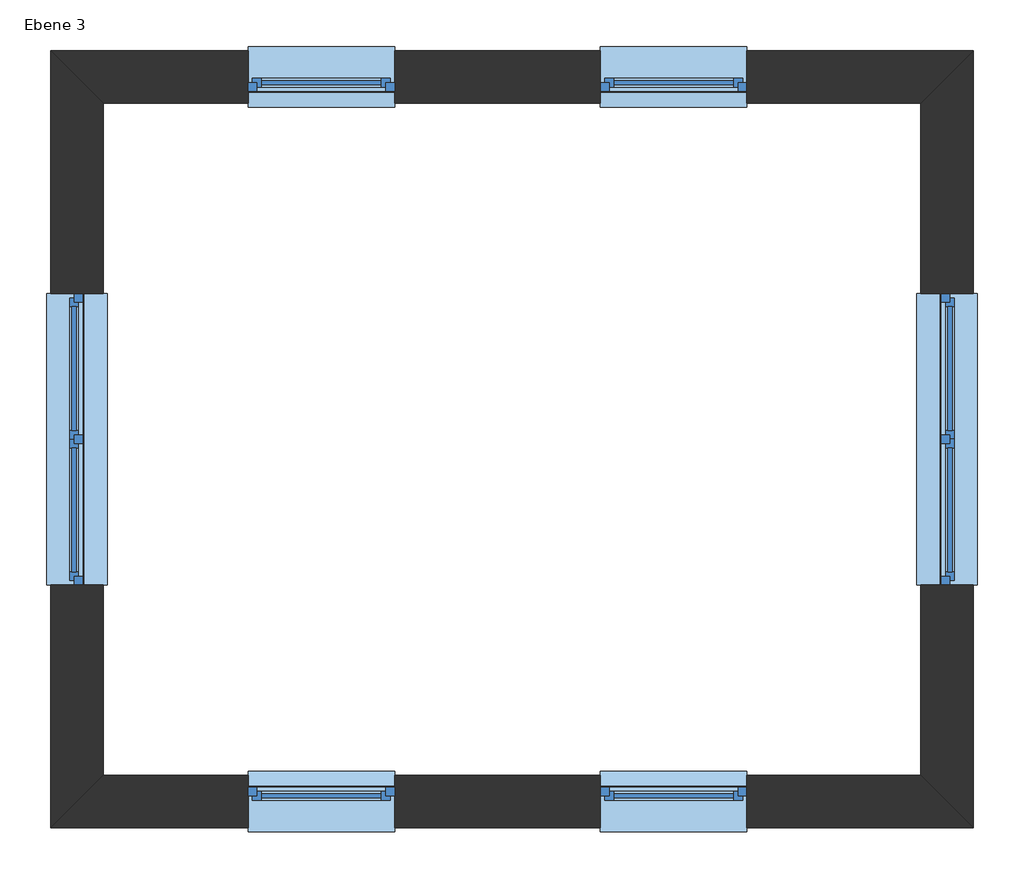
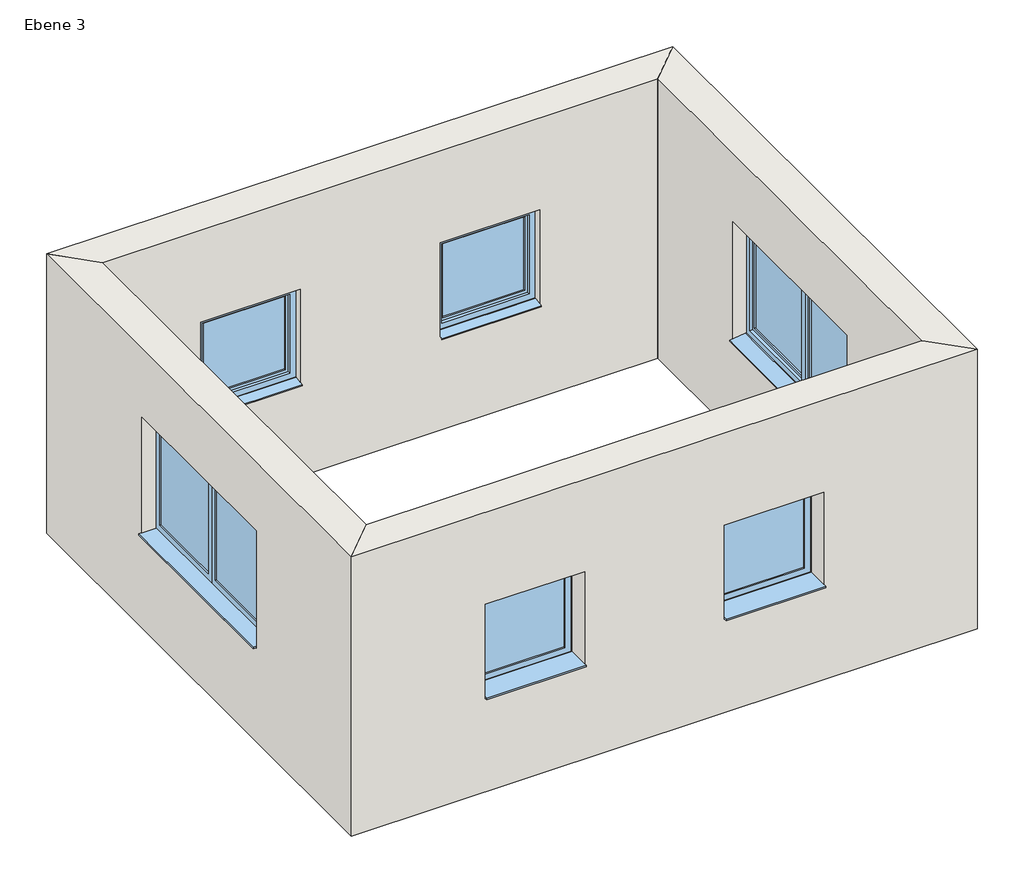
# One storey: 6 windows, 4 walls.
"""IFC4 building model written with IfcOpenShell, lengths in millimetres."""

import ifcopenshell
import ifcopenshell.guid

model = None  # the IFC model being written
_history = None  # IfcOwnerHistory: only IFC2X3 demands one
_inside = {}  # id of a spatial element -> (the spatial element, [elements in it])
_under = {}  # id of a project, library or spatial element -> (it, [spatial elements below it])
_declared = {}  # id of a project -> (the project, [libraries it declares])
_typed = {}  # id of a type object -> (the type object, [elements of that type])
_made_of = {}  # id of a material, layer set ... -> (it, [elements and type objects made of it])


def new_model(schema):
    """Start an empty IFC model of exactly this schema.

    Asked for "IFC4X3", IfcOpenShell would pick the latest addendum, in which some entities
    have other attributes; the version numbers below select the first issue.
    IFC2X3 requires an IfcOwnerHistory on every rooted entity: one is made here for all.
    """
    global model, _history
    if schema == "IFC4X3":
        model = ifcopenshell.file(schema_version=(4, 3, 0, 0))
    else:
        model = ifcopenshell.file(schema=schema)
    _inside.clear()
    _under.clear()
    _declared.clear()
    _typed.clear()
    _made_of.clear()
    _history = None
    if model.schema == "IFC2X3":
        org = make("IfcOrganization", Name="unknown")
        user = make(
            "IfcPersonAndOrganization",
            ThePerson=make("IfcPerson", FamilyName="unknown"),
            TheOrganization=org,
        )
        app = make(
            "IfcApplication",
            ApplicationDeveloper=org,
            Version="unknown",
            ApplicationFullName="unknown",
            ApplicationIdentifier="unknown",
        )
        _history = make(
            "IfcOwnerHistory",
            OwningUser=user,
            OwningApplication=app,
            ChangeAction="ADDED",
            CreationDate=0,
        )
    return model


def make(cls, **values):
    """One entity of the class cls with the attributes given. An attribute that is None is left unset."""
    return model.create_entity(
        cls, **{name: value for name, value in values.items() if value is not None}
    )


def rooted(cls, **values):
    """An entity with a GlobalId (a new one), such as an element, a storey or a relation."""
    return make(cls, GlobalId=ifcopenshell.guid.new(), OwnerHistory=_history, **values)


def si_unit(unit_type, name, prefix=None):
    """IfcSIUnit, for example si_unit("LENGTHUNIT", "METRE", prefix="MILLI")."""
    return make("IfcSIUnit", UnitType=unit_type, Prefix=prefix, Name=name)


def assignment(units):
    """IfcUnitAssignment: the units of a project."""
    return None if units is None else make("IfcUnitAssignment", Units=units)


def point(xyz):
    """IfcCartesianPoint."""
    return None if xyz is None else make("IfcCartesianPoint", Coordinates=xyz)


def direction(xyz):
    """IfcDirection."""
    return None if xyz is None else make("IfcDirection", DirectionRatios=xyz)


def frame(location, z_axis=None, x_axis=None):
    """IfcAxis2Placement3D, a coordinate frame: its origin and axes. An axis left out is left unset."""
    return make(
        "IfcAxis2Placement3D",
        Location=point(location),
        Axis=direction(z_axis),
        RefDirection=direction(x_axis),
    )


def origin():
    """The frame at (0, 0, 0) with its axes left unset."""
    return frame((0.0, 0.0, 0.0))


def place(relative_to, where):
    """IfcLocalPlacement: puts the frame where relative to a parent placement (None: the world)."""
    return make(
        "IfcLocalPlacement", PlacementRelTo=relative_to, RelativePlacement=where
    )


def context(
    kind, dimensions, precision=None, world=None, true_north=None, identifier=None
):
    """IfcGeometricRepresentationContext, for example the 3D "Model" context."""
    return make(
        "IfcGeometricRepresentationContext",
        ContextIdentifier=identifier,
        ContextType=kind,
        CoordinateSpaceDimension=dimensions,
        Precision=precision,
        WorldCoordinateSystem=world,
        TrueNorth=true_north,
    )


def project(units=None, contexts=None):
    """IfcProject with its units and contexts."""
    return rooted(
        "IfcProject",
        Name="project",
        RepresentationContexts=contexts,
        UnitsInContext=assignment(units),
    )


def spatial(cls, under=None, at=None, **own):
    """A site, building, storey or space (cls), placed at a placement, below another one or the project."""
    s = rooted(cls, ObjectPlacement=at, **own)
    if under is not None:
        _under.setdefault(under.id(), (under, []))[1].append(s)
    return s


def polyline(points):
    """IfcPolyline through the points."""
    return make("IfcPolyline", Points=[point(p) for p in points])


def outline(outer, holes=None, kind="AREA"):
    """IfcArbitraryClosedProfileDef: a profile drawn as a closed curve; with holes, ...WithVoids."""
    if holes is None:
        return make("IfcArbitraryClosedProfileDef", ProfileType=kind, OuterCurve=outer)
    return make(
        "IfcArbitraryProfileDefWithVoids",
        ProfileType=kind,
        OuterCurve=outer,
        InnerCurves=holes,
    )


def extrude(swept, where, along, depth):
    """IfcExtrudedAreaSolid: the profile swept, set in the frame where, extruded along a direction by depth."""
    return make(
        "IfcExtrudedAreaSolid",
        SweptArea=swept,
        Position=where,
        ExtrudedDirection=direction(along),
        Depth=depth,
    )


def faces_of(points, faces, orient=None, outer=None):
    """IfcFace entities. A face is a list of loops; a loop is a list of indices into points, from 0.

    orient and outer hold one flag for each loop. By default every Orientation is true, the
    first loop of a face is its IfcFaceOuterBound and the others are IfcFaceBound.
    """
    made = []
    for i, loops in enumerate(faces):
        bounds = []
        for j, loop in enumerate(loops):
            is_outer = j == 0 if outer is None else outer[i][j]
            bounds.append(
                make(
                    "IfcFaceOuterBound" if is_outer else "IfcFaceBound",
                    Bound=make("IfcPolyLoop", Polygon=[points[k] for k in loop]),
                    Orientation=True if orient is None else orient[i][j],
                )
            )
        made.append(make("IfcFace", Bounds=bounds))
    return made


def faceted_brep(points, faces, orient=None, outer=None, voids=None):
    """IfcFacetedBrep: a solid bounded by flat faces; with voids (closed shells), ...WithVoids."""
    shared = [point(p) for p in points]
    hull = make("IfcClosedShell", CfsFaces=faces_of(shared, faces, orient, outer))
    if voids is None:
        return make("IfcFacetedBrep", Outer=hull)
    return make(
        "IfcFacetedBrepWithVoids",
        Outer=hull,
        Voids=[
            make(cls, CfsFaces=faces_of(shared, fs, o, b)) for cls, fs, o, b in voids
        ],
    )


def shape(context_of_items, identifier, shape_type, items):
    """IfcShapeRepresentation: the items that make up one representation, for example the "Body"."""
    return make(
        "IfcShapeRepresentation",
        ContextOfItems=context_of_items,
        RepresentationIdentifier=identifier,
        RepresentationType=shape_type,
        Items=items,
    )


def source(mapping_origin, context_of_items, identifier, shape_type, items):
    """IfcRepresentationMap: a shape defined once, which mapped items show again and again."""
    return make(
        "IfcRepresentationMap",
        MappingOrigin=mapping_origin,
        MappedRepresentation=shape(context_of_items, identifier, shape_type, items),
    )


def transform(
    local_origin,
    x_axis=None,
    y_axis=None,
    z_axis=None,
    scale=None,
    scale2=None,
    scale3=None,
    uniform=True,
):
    """IfcCartesianTransformationOperator3D, or its non-uniform kind. x_axis, y_axis, z_axis: its Axis1, 2, 3."""
    if uniform:
        return make(
            "IfcCartesianTransformationOperator3D",
            Axis1=direction(x_axis),
            Axis2=direction(y_axis),
            LocalOrigin=point(local_origin),
            Scale=scale,
            Axis3=direction(z_axis),
        )
    return make(
        "IfcCartesianTransformationOperator3DnonUniform",
        Axis1=direction(x_axis),
        Axis2=direction(y_axis),
        LocalOrigin=point(local_origin),
        Scale=scale,
        Axis3=direction(z_axis),
        Scale2=scale2,
        Scale3=scale3,
    )


def mapped(mapping_source, mapping_target):
    """IfcMappedItem: shows the shape of a source again, moved by a transform."""
    return make(
        "IfcMappedItem", MappingSource=mapping_source, MappingTarget=mapping_target
    )


def made_of(thing, what):
    """Note that an element or type object is made of a material, layer set ...; save() writes the relation."""
    if what is not None:
        _made_of.setdefault(what.id(), (what, []))[1].append(thing)
    return thing


def element(
    cls,
    number,
    at=None,
    inside=None,
    cuts=None,
    type_object=None,
    material=None,
    context=None,
    identifier="Body",
    shape_type=None,
    held_by="IfcProductDefinitionShape",
    body=None,
    shapes=None,
    **own,
):
    """One element of the class cls, such as IfcWall. Its Tag is "e" and its number.

    at: its placement. inside: the storey or other place that contains it. cuts: it is an
    opening in that element (IfcRelVoidsElement). A single representation is given by context,
    identifier, shape_type and body (its items); several are given by shapes. held_by: the class
    of the entity that holds the representations. save() writes the other relations.
    """
    e = rooted(cls, Tag="e%d" % number, ObjectPlacement=at, **own)
    if body is not None:
        shapes = [shape(context, identifier, shape_type, body)]
    if shapes is not None:
        e.Representation = make(held_by, Representations=shapes)
    if inside is not None:
        _inside.setdefault(inside.id(), (inside, []))[1].append(e)
    if cuts is not None:
        rooted(
            "IfcRelVoidsElement", RelatingBuildingElement=cuts, RelatedOpeningElement=e
        )
    if type_object is not None:
        _typed.setdefault(type_object.id(), (type_object, []))[1].append(e)
    return made_of(e, material)


def aggregate(whole, parts):
    """IfcRelAggregates: a whole, such as a stair, and the parts it consists of."""
    return rooted("IfcRelAggregates", RelatingObject=whole, RelatedObjects=parts)


def save(model, path):
    """Write the relations noted so far, then the file.

    IfcRelAggregates (storeys below a building ...), IfcRelContainedInSpatialStructure (elements
    in a storey), IfcRelDefinesByType, IfcRelAssociatesMaterial and IfcRelDeclares: one each for
    every whole, place, type object, material and project.
    """
    for whole, parts in _under.values():
        aggregate(whole, parts)
    for where, things in _inside.values():
        rooted(
            "IfcRelContainedInSpatialStructure",
            RelatedElements=things,
            RelatingStructure=where,
        )
    for kind, things in _typed.values():
        rooted("IfcRelDefinesByType", RelatedObjects=things, RelatingType=kind)
    for what, things in _made_of.values():
        rooted("IfcRelAssociatesMaterial", RelatedObjects=things, RelatingMaterial=what)
    for by, libraries in _declared.values():
        rooted("IfcRelDeclares", RelatingContext=by, RelatedDefinitions=libraries)
    model.write(path)


def fenster_1_flg_variabel_fenster_1_flg_variabel_3_8a378bad(model_context):
    return source(origin(), model_context, "Body", "SolidModel", [
        extrude(outline(polyline([(2010.0, 505.0), (2010.0, -505.0), (1000.0, -505.0), (1000.0, 505.0), (2010.0, 505.0)]), holes=[polyline([(1930.0, 445.0), (1080.0, 445.0), (1080.0, -445.0), (1930.0, -445.0), (1930.0, 445.0)])]), frame((0.0, 40.0, 0.0), z_axis=(0.0, 1.0, 0.0), x_axis=(0.0, 0.0, 1.0)), (0.0, 0.0, 1.0), 60.0),
        faceted_brep([(475.0, 40.0, 1960.0), (475.0, 10.0, 1960.0), (475.0, 10.0, 1050.0), (475.0, 40.0, 1050.0), (-475.0, 10.0, 1960.0), (-475.0, 10.0, 1050.0), (415.0, 10.0, 1110.0), (-415.0, 10.0, 1110.0), (-415.0, 10.0, 1900.0), (415.0, 10.0, 1900.0), (-475.0, 40.0, 1050.0), (-475.0, 40.0, 1960.0), (445.0, 40.0, 1930.0), (-445.0, 40.0, 1930.0), (-445.0, 40.0, 1080.0), (445.0, 40.0, 1080.0), (445.0, 70.0, 1930.0), (445.0, 70.0, 1080.0), (-445.0, 70.0, 1080.0), (-445.0, 70.0, 1930.0), (415.0, 70.0, 1900.0), (-415.0, 70.0, 1900.0), (-415.0, 70.0, 1110.0), (415.0, 70.0, 1110.0)], [[[0, 1, 2, 3]], [[1, 4, 5, 2], [6, 7, 8, 9]], [[3, 2, 5, 10]], [[3, 10, 11, 0], [12, 13, 14, 15]], [[16, 12, 15, 17]], [[17, 15, 14, 18]], [[17, 18, 19, 16], [20, 21, 22, 23]], [[9, 20, 23, 6]], [[6, 23, 22, 7]], [[10, 5, 4, 11]], [[18, 14, 13, 19]], [[7, 22, 21, 8]], [[11, 4, 1, 0]], [[19, 13, 12, 16]], [[8, 21, 20, 9]]]),
        extrude(outline(polyline([(-505.0, -210.0), (-505.0, 40.0), (505.0, 40.0), (505.0, -210.0), (-505.0, -210.0)])), frame((0.0, 0.0, 1005.0), z_axis=(0.0, 0.0, 1.0), x_axis=(1.0, 0.0, 0.0)), (0.0, 0.0, 1.0), 15.0),
        extrude(outline(polyline([(110.0221543, 1020.0), (210.0, 1000.0), (210.0, 990.0), (208.0, 990.0), (208.0, 998.3604634), (109.8240723, 1018.0), (100.0, 1018.0), (100.0, 1020.0), (110.0221543, 1020.0)])), frame((-505.0, 0.0, 0.0), z_axis=(1.0, 0.0, 0.0), x_axis=(0.0, 1.0, 0.0)), (0.0, 0.0, 1.0), 1010.0),
        extrude(outline(polyline([(415.0, 25.0), (-415.0, 25.0), (-415.0, 55.0), (415.0, 55.0), (415.0, 25.0)])), frame((0.0, 0.0, 1110.0), z_axis=(0.0, 0.0, 1.0), x_axis=(1.0, 0.0, 0.0)), (0.0, 0.0, 1.0), 790.0),
    ])


def fenster_2_flg_variabel_fenster_2_flg_variabel_3_03287464(model_context):
    return source(origin(), model_context, "Body", "SolidModel", [
        extrude(outline(polyline([(60.0, -5.0), (915.0, -5.0), (915.0, -35.0), (60.0, -35.0), (60.0, -5.0)])), frame((0.0, 0.0, 1110.0), z_axis=(0.0, 0.0, 1.0), x_axis=(1.0, 0.0, 0.0)), (0.0, 0.0, 1.0), 1040.0),
        extrude(outline(polyline([(-915.0, -5.0), (-60.0, -5.0), (-60.0, -35.0), (-915.0, -35.0), (-915.0, -5.0)])), frame((0.0, 0.0, 1110.0), z_axis=(0.0, 0.0, 1.0), x_axis=(1.0, 0.0, 0.0)), (0.0, 0.0, 1.0), 1040.0),
        extrude(outline(polyline([(-1005.0, -210.0), (-1005.0, -20.0), (1005.0, -20.0), (1005.0, -210.0), (-1005.0, -210.0)])), frame((0.0, 0.0, 1005.0), z_axis=(0.0, 0.0, 1.0), x_axis=(1.0, 0.0, 0.0)), (0.0, 0.0, 1.0), 15.0),
        extrude(outline(polyline([(50.0221543, 1020.0), (210.0, 1000.0), (210.0, 990.0), (208.0, 990.0), (208.0, 998.3604634), (49.8240723, 1018.0), (40.0, 1018.0), (40.0, 1020.0), (50.0221543, 1020.0)])), frame((-1005.0, 0.0, 0.0), z_axis=(1.0, 0.0, 0.0), x_axis=(0.0, 1.0, 0.0)), (0.0, 0.0, 1.0), 2010.0),
        extrude(outline(polyline([(30.0, -20.0), (-30.0, -20.0), (-30.0, 40.0), (30.0, 40.0), (30.0, -20.0)])), frame((0.0, 0.0, 1080.0), z_axis=(0.0, 0.0, 1.0), x_axis=(1.0, 0.0, 0.0)), (0.0, 0.0, 1.0), 1100.0),
        extrude(outline(polyline([(2260.0, -1005.0), (1000.0, -1005.0), (1000.0, 1005.0), (2260.0, 1005.0), (2260.0, -1005.0)]), holes=[polyline([(2180.0, -945.0), (2180.0, 945.0), (1080.0, 945.0), (1080.0, -945.0), (2180.0, -945.0)])]), frame((0.0, -20.0, 0.0), z_axis=(0.0, 1.0, 0.0), x_axis=(0.0, 0.0, 1.0)), (0.0, 0.0, 1.0), 60.0),
        faceted_brep([(-945.0, -20.0, 1080.0), (-945.0, 10.0, 1080.0), (-30.0, 10.0, 1080.0), (-30.0, -20.0, 1080.0), (-30.0, 10.0, 2180.0), (-30.0, -20.0, 2180.0), (-945.0, 10.0, 2180.0), (-60.0, 10.0, 2150.0), (-915.0, 10.0, 2150.0), (-915.0, 10.0, 1110.0), (-60.0, 10.0, 1110.0), (0.0, -20.0, 1050.0), (-975.0, -20.0, 1050.0), (-975.0, -20.0, 2210.0), (0.0, -20.0, 2210.0), (-945.0, -20.0, 2180.0), (-975.0, -50.0, 1050.0), (0.0, -50.0, 1050.0), (0.0, -50.0, 2210.0), (-975.0, -50.0, 2210.0), (-60.0, -50.0, 1110.0), (-915.0, -50.0, 1110.0), (-915.0, -50.0, 2150.0), (-60.0, -50.0, 2150.0)], [[[0, 1, 2, 3]], [[3, 2, 4, 5]], [[2, 1, 6, 4], [7, 8, 9, 10]], [[11, 12, 13, 14], [5, 15, 0, 3]], [[16, 12, 11, 17]], [[17, 11, 14, 18]], [[18, 19, 16, 17], [20, 21, 22, 23]], [[9, 21, 20, 10]], [[10, 20, 23, 7]], [[15, 6, 1, 0]], [[19, 13, 12, 16]], [[8, 22, 21, 9]], [[5, 4, 6, 15]], [[18, 14, 13, 19]], [[7, 23, 22, 8]]]),
        faceted_brep([(30.0, -20.0, 1080.0), (30.0, 10.0, 1080.0), (945.0, 10.0, 1080.0), (945.0, -20.0, 1080.0), (945.0, 10.0, 2180.0), (945.0, -20.0, 2180.0), (30.0, 10.0, 2180.0), (915.0, 10.0, 2150.0), (60.0, 10.0, 2150.0), (60.0, 10.0, 1110.0), (915.0, 10.0, 1110.0), (975.0, -20.0, 1050.0), (0.0, -20.0, 1050.0), (0.0, -20.0, 2210.0), (975.0, -20.0, 2210.0), (30.0, -20.0, 2180.0), (0.0, -50.0, 1050.0), (975.0, -50.0, 1050.0), (975.0, -50.0, 2210.0), (0.0, -50.0, 2210.0), (915.0, -50.0, 1110.0), (60.0, -50.0, 1110.0), (60.0, -50.0, 2150.0), (915.0, -50.0, 2150.0)], [[[0, 1, 2, 3]], [[3, 2, 4, 5]], [[2, 1, 6, 4], [7, 8, 9, 10]], [[11, 12, 13, 14], [5, 15, 0, 3]], [[16, 12, 11, 17]], [[17, 11, 14, 18]], [[18, 19, 16, 17], [20, 21, 22, 23]], [[9, 21, 20, 10]], [[10, 20, 23, 7]], [[15, 6, 1, 0]], [[19, 13, 12, 16]], [[8, 22, 21, 9]], [[5, 4, 6, 15]], [[18, 14, 13, 19]], [[7, 23, 22, 8]]]),
    ])


model = new_model("IFC4")

# Units and contexts
model_context = context("Model", 3, world=origin())
ifc_project = project(units=[si_unit("LENGTHUNIT", "METRE", prefix="MILLI")], contexts=[model_context])

# Site, building, storey
site = spatial("IfcSite", under=ifc_project)
building = spatial("IfcBuilding", under=site)
storey = spatial("IfcBuildingStorey", under=building, Name="Ebene 3", Elevation=9000.0)

# Walls
placement = place(None, origin())
element("IfcWall", 1, ObjectType="MW 24.0 WD 12.0", at=placement, inside=storey, context=model_context, shape_type="Brep", body=[
    faceted_brep([(-3766.4979049, 4044.3692517, 9000.0), (1873.5020951, 4044.3692517, 9000.0), (1873.5020951, 4044.3692517, 12000.0), (-3766.4979049, 4044.3692517, 12000.0), (673.5020951, 4044.3692517, 10000.0), (-336.4979049, 4044.3692517, 10000.0), (-336.4979049, 4044.3692517, 11010.0), (673.5020951, 4044.3692517, 11010.0), (-1756.4979049, 4044.3692517, 10000.0), (-2766.4979049, 4044.3692517, 10000.0), (-2766.4979049, 4044.3692517, 11010.0), (-1756.4979049, 4044.3692517, 11010.0), (-4126.4979049, 4404.3692517, 9000.0), (-4126.4979049, 4404.3692517, 12000.0), (2233.5020951, 4404.3692517, 12000.0), (2233.5020951, 4404.3692517, 9000.0), (673.5020951, 4404.3692517, 10000.0), (673.5020951, 4404.3692517, 11010.0), (-336.4979049, 4404.3692517, 11010.0), (-336.4979049, 4404.3692517, 10000.0), (-1756.4979049, 4404.3692517, 10000.0), (-1756.4979049, 4404.3692517, 11010.0), (-2766.4979049, 4404.3692517, 11010.0), (-2766.4979049, 4404.3692517, 10000.0)], [[[0, 1, 2, 3], [4, 5, 6, 7], [8, 9, 10, 11]], [[12, 13, 14, 15], [16, 17, 18, 19], [20, 21, 22, 23]], [[1, 0, 12, 15]], [[3, 2, 14, 13]], [[2, 1, 15, 14]], [[0, 3, 13, 12]], [[17, 16, 4, 7]], [[18, 17, 7, 6]], [[19, 18, 6, 5]], [[16, 19, 5, 4]], [[21, 20, 8, 11]], [[22, 21, 11, 10]], [[23, 22, 10, 9]], [[20, 23, 9, 8]]]),
])
element("IfcWall", 2, ObjectType="MW 24.0 WD 12.0", at=placement, inside=storey, context=model_context, shape_type="Brep", body=[
    faceted_brep([(1873.5020951, 4044.3692517, 9000.0), (1873.5020951, -595.6307483, 9000.0), (1873.5020951, -595.6307483, 12000.0), (1873.5020951, 4044.3692517, 12000.0), (1873.5020951, 719.3692517, 10000.0), (1873.5020951, 2729.3692517, 10000.0), (1873.5020951, 2729.3692517, 11260.0), (1873.5020951, 719.3692517, 11260.0), (2233.5020951, 4404.3692517, 9000.0), (2233.5020951, 4404.3692517, 12000.0), (2233.5020951, -955.6307483, 12000.0), (2233.5020951, -955.6307483, 9000.0), (2233.5020951, 719.3692517, 10000.0), (2233.5020951, 719.3692517, 11260.0), (2233.5020951, 2729.3692517, 11260.0), (2233.5020951, 2729.3692517, 10000.0)], [[[0, 1, 2, 3], [4, 5, 6, 7]], [[8, 9, 10, 11], [12, 13, 14, 15]], [[1, 0, 8, 11]], [[3, 2, 10, 9]], [[0, 3, 9, 8]], [[2, 1, 11, 10]], [[13, 12, 4, 7]], [[14, 13, 7, 6]], [[15, 14, 6, 5]], [[12, 15, 5, 4]]]),
])
element("IfcWall", 3, ObjectType="MW 24.0 WD 12.0", at=placement, inside=storey, context=model_context, shape_type="Brep", body=[
    faceted_brep([(1873.5020951, -595.6307483, 9000.0), (-3766.4979049, -595.6307483, 9000.0), (-3766.4979049, -595.6307483, 12000.0), (1873.5020951, -595.6307483, 12000.0), (-336.4979049, -595.6307483, 10000.0), (673.5020951, -595.6307483, 10000.0), (673.5020951, -595.6307483, 11010.0), (-336.4979049, -595.6307483, 11010.0), (-2766.4979049, -595.6307483, 10000.0), (-1756.4979049, -595.6307483, 10000.0), (-1756.4979049, -595.6307483, 11010.0), (-2766.4979049, -595.6307483, 11010.0), (2233.5020951, -955.6307483, 9000.0), (2233.5020951, -955.6307483, 12000.0), (-4126.4979049, -955.6307483, 12000.0), (-4126.4979049, -955.6307483, 9000.0), (-336.4979049, -955.6307483, 10000.0), (-336.4979049, -955.6307483, 11010.0), (673.5020951, -955.6307483, 11010.0), (673.5020951, -955.6307483, 10000.0), (-2766.4979049, -955.6307483, 10000.0), (-2766.4979049, -955.6307483, 11010.0), (-1756.4979049, -955.6307483, 11010.0), (-1756.4979049, -955.6307483, 10000.0)], [[[0, 1, 2, 3], [4, 5, 6, 7], [8, 9, 10, 11]], [[12, 13, 14, 15], [16, 17, 18, 19], [20, 21, 22, 23]], [[1, 0, 12, 15]], [[3, 2, 14, 13]], [[0, 3, 13, 12]], [[2, 1, 15, 14]], [[17, 16, 4, 7]], [[18, 17, 7, 6]], [[19, 18, 6, 5]], [[16, 19, 5, 4]], [[21, 20, 8, 11]], [[22, 21, 11, 10]], [[23, 22, 10, 9]], [[20, 23, 9, 8]]]),
])
element("IfcWall", 4, ObjectType="MW 24.0 WD 12.0", at=placement, inside=storey, context=model_context, shape_type="Brep", body=[
    faceted_brep([(-3766.4979049, -595.6307483, 9000.0), (-3766.4979049, 4044.3692517, 9000.0), (-3766.4979049, 4044.3692517, 12000.0), (-3766.4979049, -595.6307483, 12000.0), (-3766.4979049, 2729.3692517, 10000.0), (-3766.4979049, 719.3692517, 10000.0), (-3766.4979049, 719.3692517, 11260.0), (-3766.4979049, 2729.3692517, 11260.0), (-4126.4979049, -955.6307483, 9000.0), (-4126.4979049, -955.6307483, 12000.0), (-4126.4979049, 4404.3692517, 12000.0), (-4126.4979049, 4404.3692517, 9000.0), (-4126.4979049, 2729.3692517, 10000.0), (-4126.4979049, 2729.3692517, 11260.0), (-4126.4979049, 719.3692517, 11260.0), (-4126.4979049, 719.3692517, 10000.0)], [[[0, 1, 2, 3], [4, 5, 6, 7]], [[8, 9, 10, 11], [12, 13, 14, 15]], [[1, 0, 8, 11]], [[3, 2, 10, 9]], [[2, 1, 11, 10]], [[0, 3, 9, 8]], [[13, 12, 4, 7]], [[14, 13, 7, 6]], [[15, 14, 6, 5]], [[12, 15, 5, 4]]]),
])

# Windows
fenster_1_flg_variabel_fenster_1_flg_variabel_3_shape = fenster_1_flg_variabel_fenster_1_flg_variabel_3_8a378bad(model_context)
element("IfcWindow", 5, ObjectType="Fenster 1-flg - Variabel : Fenster 1-flg - Variabel 3", at=placement, inside=storey, context=model_context, shape_type="MappedRepresentation", body=[
    mapped(fenster_1_flg_variabel_fenster_1_flg_variabel_3_shape, transform((168.5020951, -775.6307483, 9000.0), x_axis=(1.0, 0.0, 0.0), y_axis=(0.0, 1.0, 0.0), z_axis=(0.0, 0.0, 1.0))),
])
element("IfcWindow", 6, ObjectType="Fenster 1-flg - Variabel : Fenster 1-flg - Variabel 3", at=placement, inside=storey, context=model_context, shape_type="MappedRepresentation", body=[
    mapped(fenster_1_flg_variabel_fenster_1_flg_variabel_3_shape, transform((-2261.4979049, -775.6307483, 9000.0), x_axis=(1.0, 0.0, 0.0), y_axis=(0.0, 1.0, 0.0), z_axis=(0.0, 0.0, 1.0))),
])
element("IfcWindow", 7, ObjectType="Fenster 1-flg - Variabel : Fenster 1-flg - Variabel 3", at=placement, inside=storey, context=model_context, shape_type="MappedRepresentation", body=[
    mapped(fenster_1_flg_variabel_fenster_1_flg_variabel_3_shape, transform((168.5020951, 4224.3692517, 9000.0), x_axis=(-1.0, 0.0, 0.0), y_axis=(0.0, -1.0, 0.0), z_axis=(0.0, 0.0, 1.0))),
])
element("IfcWindow", 8, ObjectType="Fenster 1-flg - Variabel : Fenster 1-flg - Variabel 3", at=placement, inside=storey, context=model_context, shape_type="MappedRepresentation", body=[
    mapped(fenster_1_flg_variabel_fenster_1_flg_variabel_3_shape, transform((-2261.4979049, 4224.3692517, 9000.0), x_axis=(-1.0, 0.0, 0.0), y_axis=(0.0, -1.0, 0.0), z_axis=(0.0, 0.0, 1.0))),
])
fenster_2_flg_variabel_fenster_2_flg_variabel_3_shape = fenster_2_flg_variabel_fenster_2_flg_variabel_3_03287464(model_context)
element("IfcWindow", 9, ObjectType="Fenster 2-flg - Variabel : Fenster 2-flg - Variabel 3", at=placement, inside=storey, context=model_context, shape_type="MappedRepresentation", body=[
    mapped(fenster_2_flg_variabel_fenster_2_flg_variabel_3_shape, transform((2053.5020951, 1724.3692517, 9000.0), x_axis=(0.0, 1.0, 0.0), y_axis=(-1.0, 0.0, 0.0), z_axis=(0.0, 0.0, 1.0))),
])
element("IfcWindow", 10, ObjectType="Fenster 2-flg - Variabel : Fenster 2-flg - Variabel 3", at=placement, inside=storey, context=model_context, shape_type="MappedRepresentation", body=[
    mapped(fenster_2_flg_variabel_fenster_2_flg_variabel_3_shape, transform((-3946.4979049, 1724.3692517, 9000.0), x_axis=(0.0, -1.0, 0.0), y_axis=(1.0, 0.0, 0.0), z_axis=(0.0, 0.0, 1.0))),
])

save(model, "model.ifc")

# Revit data of these elements
# Type "MW 24.0 WD 12.0"
#   Type Comments = "Mehrschaliges Mauerwerk"
#   Description = "Mauerwerk 24.0 cm, Wärmedämmung 12.0 cm"
#   Layers, outside or top first: 0.120 m "Wärmedämmung - hart" (function 3); 0.240 m "Mauerwerk - Ziegel, verputzt" (function 1)
# Type "Fenster 1-flg - Variabel : Fenster 1-flg - Variabel 3"
#   Type Mark = "52"
#   Operation = "SinglePanel"
#   Construction Type Id = "GSP4R"
#   Keynote = "16.05.01"
#   Analytic Construction = "1/8 Zoll Pilkington-Verglasung einfach"
#   Cost = 78.2
#   Visual Light Transmittance = 0.9
#   Höhe oberer  Rahmen = 0.080 m
#   Solar Heat Gain Coefficient = 0.86
#   Tiefe Flügel = 0.060 m
#   Rough Width [instance default] = 1.010 m
#   Rough Height [instance default] = 1.010 m
#   Rahmenhöhe unten = 0.080 m
#   Heat Transfer Coefficient (U) = 6.7069 W/(m²·K)
#   Rahmentiefe = 0.060 m
#   Rahmenbreite = 0.060 m
#   Height [instance default] = 1.010 m
#   Flügelbreite = 0.060 m
#   Einbautiefe (von außen) [instance default] = 0.080 m
#   Width [instance default] = 1.010 m
#   Define Thermal Properties by = 1
#   Öffnungsrichtung oben [instance default] = yes
#   Öffnungsrichtung in Draufsicht anzeigen [instance default] = no
#   Klappflügel [instance default] = no
#   Drehflügel 1 [instance default] = yes
#   Fensterflügel [instance default] = none
#   Innere Fensterbank [instance default] = none
#   Glas [instance default] = none
#   Bild [instance default] = none
#   Äußere Fensterbank [instance default] = none
#   Wall Closure = (empty or 0)
# Type "Fenster 2-flg - Variabel : Fenster 2-flg - Variabel 3"
#   Type Mark = "53"
#   Operation = "DoublePanelVertical"
#   Construction Type Id = "GSP4R"
#   Keynote = "16.05.01"
#   Analytic Construction = "1/8 Zoll Pilkington-Verglasung einfach"
#   Cost = 130.98
#   Visual Light Transmittance = 0.9
#   Solar Heat Gain Coefficient = 0.78
#   Rough Width [instance default] = 2.010 m
#   Rough Height [instance default] = 1.260 m
#   Heat Transfer Coefficient (U) = 3.6886 W/(m²·K)
#   Rahmentiefe = 0.060 m
#   Rahmenhöhe unten = 0.080 m
#   Höhe oberer  Rahmen = 0.080 m
#   Rahmenbreite = 0.060 m
#   Height [instance default] = 1.260 m
#   Tiefe Flügel = 0.060 m
#   Flügelbreite = 0.060 m
#   Einbautiefe (von außen) [instance default] = 0.140 m
#   Width [instance default] = 2.010 m
#   Define Thermal Properties by = 1
#   Öffnungsrichtung oben [instance default] = yes
#   Öffnungsrichtung in Draufsicht anzeigen [instance default] = no
#   Drehflügel 1 [instance default] = yes
#   Bild [instance default] = none
#   Glas [instance default] = none
#   Fensterflügel [instance default] = none
#   Äußere Fensterbank [instance default] = none
#   Innere Fensterbank [instance default] = none
#   Wall Closure = (empty or 0)
# Elements 1, 2, 3, 4 (IfcWall, "MW 24.0 WD 12.0")
#   Comments = ""
#   Top Offset = 0.000 m
#   Base Offset = 0.000 m
#   Unconnected Height = 3.000 m
#   wall height = 3.000 m
#   Phase Created = Phase 1
#   Base Constraint = Ebene 3
#   Materials on its faces: "Vorgabe - Wand", "Mauerwerk - Ziegel, verputzt", "Wärmedämmung - hart"
# Element 5 (IfcWindow, "Fenster 1-flg - Variabel : Fenster 1-flg - Variabel 3")
#   Mark = "16"
#   Rough Height = 1.010 m
#   Rough Width = 1.010 m
#   Height = 1.010 m
#   Einbautiefe (von außen) = 0.080 m
#   Width = 1.010 m
#   Öffnungsrichtung oben = yes
#   Öffnungsrichtung in Draufsicht anzeigen = no
#   Klappflügel = no
#   Drehflügel 1 = yes
#   Äußere Fensterbank = none
#   Innere Fensterbank = none
#   Glas = none
#   Fensterflügel = none
#   Bild = none
#   Phase Created = Phase 1
#   Materials on its faces: "Kunststoff - Weiß", "Holz - Birke", "Glas"
# Element 6 (IfcWindow, "Fenster 1-flg - Variabel : Fenster 1-flg - Variabel 3")
#   Mark = "17"
#   Rough Height = 1.010 m
#   Rough Width = 1.010 m
#   Height = 1.010 m
#   Einbautiefe (von außen) = 0.080 m
#   Width = 1.010 m
#   Öffnungsrichtung oben = yes
#   Öffnungsrichtung in Draufsicht anzeigen = no
#   Klappflügel = no
#   Drehflügel 1 = yes
#   Äußere Fensterbank = none
#   Innere Fensterbank = none
#   Glas = none
#   Fensterflügel = none
#   Bild = none
#   Phase Created = Phase 1
#   Materials on its faces: "Kunststoff - Weiß", "Holz - Birke", "Glas"
# Element 7 (IfcWindow, "Fenster 1-flg - Variabel : Fenster 1-flg - Variabel 3")
#   Mark = "18"
#   Rough Height = 1.010 m
#   Rough Width = 1.010 m
#   Height = 1.010 m
#   Einbautiefe (von außen) = 0.080 m
#   Width = 1.010 m
#   Öffnungsrichtung oben = yes
#   Öffnungsrichtung in Draufsicht anzeigen = no
#   Klappflügel = no
#   Drehflügel 1 = yes
#   Äußere Fensterbank = none
#   Innere Fensterbank = none
#   Glas = none
#   Fensterflügel = none
#   Bild = none
#   Phase Created = Phase 1
#   Materials on its faces: "Kunststoff - Weiß", "Holz - Birke", "Glas"
# Element 8 (IfcWindow, "Fenster 1-flg - Variabel : Fenster 1-flg - Variabel 3")
#   Mark = "19"
#   Rough Height = 1.010 m
#   Rough Width = 1.010 m
#   Height = 1.010 m
#   Einbautiefe (von außen) = 0.080 m
#   Width = 1.010 m
#   Öffnungsrichtung oben = yes
#   Öffnungsrichtung in Draufsicht anzeigen = no
#   Klappflügel = no
#   Drehflügel 1 = yes
#   Äußere Fensterbank = none
#   Innere Fensterbank = none
#   Glas = none
#   Fensterflügel = none
#   Bild = none
#   Phase Created = Phase 1
#   Materials on its faces: "Kunststoff - Weiß", "Holz - Birke", "Glas"
# Element 9 (IfcWindow, "Fenster 2-flg - Variabel : Fenster 2-flg - Variabel 3")
#   Mark = "20"
#   Rough Height = 1.260 m
#   Rough Width = 2.010 m
#   Height = 1.260 m
#   Einbautiefe (von außen) = 0.140 m
#   Width = 2.010 m
#   Öffnungsrichtung oben = yes
#   Öffnungsrichtung in Draufsicht anzeigen = no
#   Drehflügel 1 = yes
#   Äußere Fensterbank = none
#   Innere Fensterbank = none
#   Glas = none
#   Fensterflügel = none
#   Bild = none
#   Phase Created = Phase 1
#   Materials on its faces: "Kunststoff - Weiß", "Glas", "Holz - Birke"
# Element 10 (IfcWindow, "Fenster 2-flg - Variabel : Fenster 2-flg - Variabel 3")
#   Mark = "21"
#   Rough Height = 1.260 m
#   Rough Width = 2.010 m
#   Height = 1.260 m
#   Einbautiefe (von außen) = 0.140 m
#   Width = 2.010 m
#   Öffnungsrichtung oben = yes
#   Öffnungsrichtung in Draufsicht anzeigen = no
#   Drehflügel 1 = yes
#   Äußere Fensterbank = none
#   Innere Fensterbank = none
#   Glas = none
#   Fensterflügel = none
#   Bild = none
#   Phase Created = Phase 1
#   Materials on its faces: "Kunststoff - Weiß", "Glas", "Holz - Birke"
# Materials
#   "Wärmedämmung - hart": class "Stuck", colour RGB 255 255 255, transparency 0, Description = "Äußere Oberfläche", Cost = 0
#   "Mauerwerk - Ziegel, verputzt": class "Stuck", colour RGB 247 247 247, transparency 0, Cost = 0
#   "Vorgabe - Wand": class "Stuck", colour RGB 128 128 128, transparency 0, Description = "Äußere Oberfläche", Cost = 0
#   "Kunststoff - Weiß": class "Kunststoff", colour RGB 249 249 249, transparency 0, Cost = 0
#   "Holz - Birke": class "Holz", colour RGB 213 164 103, transparency 0, Cost = 0
#   "Glas": class "Glas", colour RGB 0 0 255, transparency 0.75, Comments = "Render-Darstellung nicht aktualisiert ", Cost = 0
